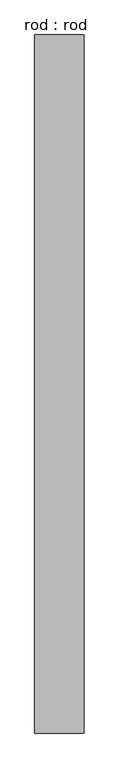
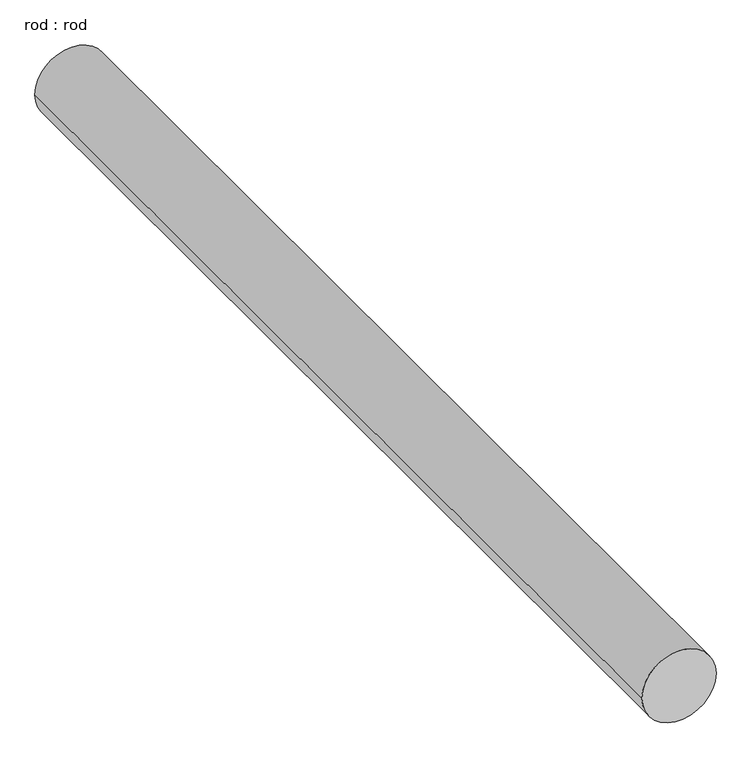
"""IFC4 building model written with IfcOpenShell, lengths in millimetres: proxy geometry, rod : rod."""

from ifc_helpers import new_model, si_unit, point, frame, frame_2d, origin, place, context, project, spatial, circle_curve, trimmed, segment, composite_curve, outline, extrude, source, transform, mapped, element, save


def rod_rod_1bf74396(model_context):
    return source(origin(), model_context, "Body", "SweptSolid", [
        extrude(outline(composite_curve([segment(trimmed(circle_curve(frame_2d((0.0108462, 0.0)), 200.0), [point((0.0108462, 200.0))], [point((0.0108462, -200.0))], False, "CARTESIAN"), True, "CONTINUOUS"), segment(trimmed(circle_curve(frame_2d((0.0108462, 0.0)), 200.0), [point((0.0108462, -200.0))], [point((0.0108462, 200.0))], False, "CARTESIAN"), True, "CONTINUOUS")], self_intersect=False)), frame((0.0, 1254.1383816, 0.0), z_axis=(0.0, 1.0, 0.0), x_axis=(0.0, 0.0, 1.0)), (0.0, 0.0, 1.0), 5677.1804676),
    ])


if __name__ == "__main__":
    model = new_model("IFC4")
    model_context = context("Model", 3, world=origin())
    ifc_project = project(units=[si_unit("LENGTHUNIT", "METRE", prefix="MILLI")], contexts=[model_context])
    site = spatial("IfcSite", under=ifc_project)
    building = spatial("IfcBuilding", under=site)
    placement = place(None, origin())
    rod_rod_shape = rod_rod_1bf74396(model_context)
    element("IfcBuildingElementProxy", 1, Name="rod : rod", ObjectType="rod : rod", at=placement, inside=building, context=model_context, shape_type="MappedRepresentation", body=[
        mapped(rod_rod_shape, transform((0.0, 0.0, 0.0), x_axis=(1.0, 0.0, 0.0), y_axis=(0.0, 1.0, 0.0), z_axis=(0.0, 0.0, 1.0))),
    ])
    save(model, "model.ifc")

# Revit data of these elements
# Type "rod : rod"
#   Default Elevation = 0
